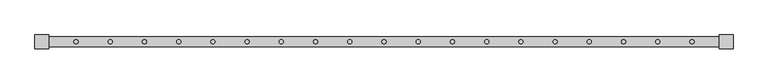
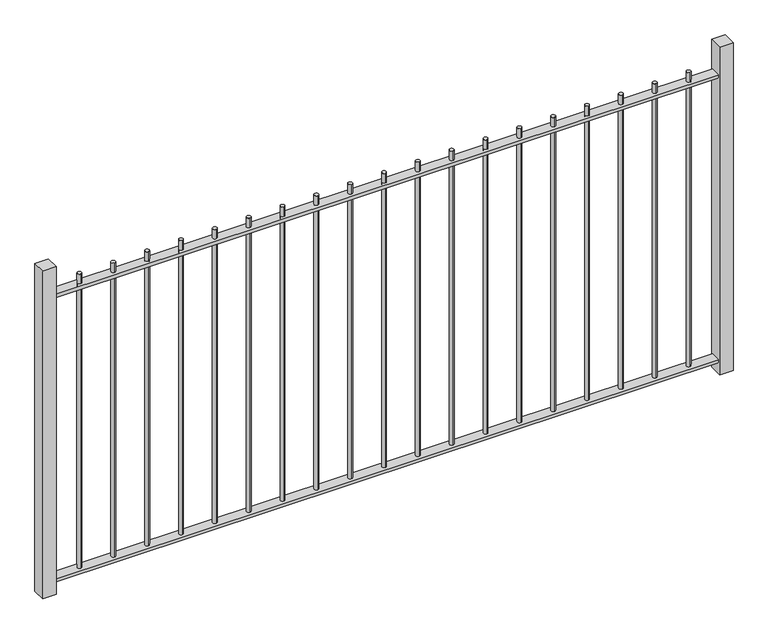
"""IFC4 building model written with IfcOpenShell, lengths in millimetres: railing geometry."""

from ifc_helpers import new_model, si_unit, point, frame, frame_2d, origin, place, context, project, spatial, polyline, circle_curve, trimmed, segment, composite_curve, outline, extrude, source, transform, mapped, element, save


def railing_b2c4460c(model_context):
    return source(origin(), model_context, "Body", "SweptSolid", [
        extrude(outline(polyline([(8650.4300877, -24901.1119119), (8650.4300877, -24961.1119119), (4650.4300877, -24961.1119119), (4650.4300877, -24901.1119119), (8650.4300877, -24901.1119119)])), frame((0.0, 0.0, -30.0), z_axis=(0.0, 0.0, 1.0), x_axis=(1.0, 0.0, 0.0)), (0.0, 0.0, 1.0), 20.0),
        extrude(outline(polyline([(8650.4300877, -24901.1119119), (8650.4300877, -24961.1119119), (4650.4300877, -24961.1119119), (4650.4300877, -24901.1119119), (8650.4300877, -24901.1119119)])), frame((0.0, 0.0, 1750.0), z_axis=(0.0, 0.0, 1.0), x_axis=(1.0, 0.0, 0.0)), (0.0, 0.0, 1.0), 20.0),
        extrude(outline(composite_curve([segment(trimmed(circle_curve(frame_2d((4850.4300877, -24931.1119119)), 12.5), [point((4850.4300877, -24943.6119119))], [point((4850.4300877, -24918.6119119))], False, "CARTESIAN"), True, "CONTINUOUS"), segment(trimmed(circle_curve(frame_2d((4850.4300877, -24931.1119119)), 12.5), [point((4850.4300877, -24918.6119119))], [point((4850.4300877, -24943.6119119))], False, "CARTESIAN"), True, "CONTINUOUS")], self_intersect=False)), frame((0.0, 0.0, -10.0), z_axis=(0.0, 0.0, 1.0), x_axis=(1.0, 0.0, 0.0)), (0.0, 0.0, 1.0), 1840.0),
        extrude(outline(composite_curve([segment(trimmed(circle_curve(frame_2d((5050.4300877, -24931.1119119)), 12.5), [point((5050.4300877, -24943.6119119))], [point((5050.4300877, -24918.6119119))], False, "CARTESIAN"), True, "CONTINUOUS"), segment(trimmed(circle_curve(frame_2d((5050.4300877, -24931.1119119)), 12.5), [point((5050.4300877, -24918.6119119))], [point((5050.4300877, -24943.6119119))], False, "CARTESIAN"), True, "CONTINUOUS")], self_intersect=False)), frame((0.0, 0.0, -10.0), z_axis=(0.0, 0.0, 1.0), x_axis=(1.0, 0.0, 0.0)), (0.0, 0.0, 1.0), 1840.0),
        extrude(outline(composite_curve([segment(trimmed(circle_curve(frame_2d((5250.4300877, -24931.1119119)), 12.5), [point((5250.4300877, -24943.6119119))], [point((5250.4300877, -24918.6119119))], False, "CARTESIAN"), True, "CONTINUOUS"), segment(trimmed(circle_curve(frame_2d((5250.4300877, -24931.1119119)), 12.5), [point((5250.4300877, -24918.6119119))], [point((5250.4300877, -24943.6119119))], False, "CARTESIAN"), True, "CONTINUOUS")], self_intersect=False)), frame((0.0, 0.0, -10.0), z_axis=(0.0, 0.0, 1.0), x_axis=(1.0, 0.0, 0.0)), (0.0, 0.0, 1.0), 1840.0),
        extrude(outline(composite_curve([segment(trimmed(circle_curve(frame_2d((5450.4300877, -24931.1119119)), 12.5), [point((5450.4300877, -24943.6119119))], [point((5450.4300877, -24918.6119119))], False, "CARTESIAN"), True, "CONTINUOUS"), segment(trimmed(circle_curve(frame_2d((5450.4300877, -24931.1119119)), 12.5), [point((5450.4300877, -24918.6119119))], [point((5450.4300877, -24943.6119119))], False, "CARTESIAN"), True, "CONTINUOUS")], self_intersect=False)), frame((0.0, 0.0, -10.0), z_axis=(0.0, 0.0, 1.0), x_axis=(1.0, 0.0, 0.0)), (0.0, 0.0, 1.0), 1840.0),
        extrude(outline(composite_curve([segment(trimmed(circle_curve(frame_2d((5650.4300877, -24931.1119119)), 12.5), [point((5650.4300877, -24943.6119119))], [point((5650.4300877, -24918.6119119))], False, "CARTESIAN"), True, "CONTINUOUS"), segment(trimmed(circle_curve(frame_2d((5650.4300877, -24931.1119119)), 12.5), [point((5650.4300877, -24918.6119119))], [point((5650.4300877, -24943.6119119))], False, "CARTESIAN"), True, "CONTINUOUS")], self_intersect=False)), frame((0.0, 0.0, -10.0), z_axis=(0.0, 0.0, 1.0), x_axis=(1.0, 0.0, 0.0)), (0.0, 0.0, 1.0), 1840.0),
        extrude(outline(composite_curve([segment(trimmed(circle_curve(frame_2d((5850.4300877, -24931.1119119)), 12.5), [point((5850.4300877, -24943.6119119))], [point((5850.4300877, -24918.6119119))], False, "CARTESIAN"), True, "CONTINUOUS"), segment(trimmed(circle_curve(frame_2d((5850.4300877, -24931.1119119)), 12.5), [point((5850.4300877, -24918.6119119))], [point((5850.4300877, -24943.6119119))], False, "CARTESIAN"), True, "CONTINUOUS")], self_intersect=False)), frame((0.0, 0.0, -10.0), z_axis=(0.0, 0.0, 1.0), x_axis=(1.0, 0.0, 0.0)), (0.0, 0.0, 1.0), 1840.0),
        extrude(outline(composite_curve([segment(trimmed(circle_curve(frame_2d((6050.4300877, -24931.1119119)), 12.5), [point((6050.4300877, -24943.6119119))], [point((6050.4300877, -24918.6119119))], False, "CARTESIAN"), True, "CONTINUOUS"), segment(trimmed(circle_curve(frame_2d((6050.4300877, -24931.1119119)), 12.5), [point((6050.4300877, -24918.6119119))], [point((6050.4300877, -24943.6119119))], False, "CARTESIAN"), True, "CONTINUOUS")], self_intersect=False)), frame((0.0, 0.0, -10.0), z_axis=(0.0, 0.0, 1.0), x_axis=(1.0, 0.0, 0.0)), (0.0, 0.0, 1.0), 1840.0),
        extrude(outline(composite_curve([segment(trimmed(circle_curve(frame_2d((6250.4300877, -24931.1119119)), 12.5), [point((6250.4300877, -24943.6119119))], [point((6250.4300877, -24918.6119119))], False, "CARTESIAN"), True, "CONTINUOUS"), segment(trimmed(circle_curve(frame_2d((6250.4300877, -24931.1119119)), 12.5), [point((6250.4300877, -24918.6119119))], [point((6250.4300877, -24943.6119119))], False, "CARTESIAN"), True, "CONTINUOUS")], self_intersect=False)), frame((0.0, 0.0, -10.0), z_axis=(0.0, 0.0, 1.0), x_axis=(1.0, 0.0, 0.0)), (0.0, 0.0, 1.0), 1840.0),
        extrude(outline(composite_curve([segment(trimmed(circle_curve(frame_2d((6450.4300877, -24931.1119119)), 12.5), [point((6450.4300877, -24943.6119119))], [point((6450.4300877, -24918.6119119))], False, "CARTESIAN"), True, "CONTINUOUS"), segment(trimmed(circle_curve(frame_2d((6450.4300877, -24931.1119119)), 12.5), [point((6450.4300877, -24918.6119119))], [point((6450.4300877, -24943.6119119))], False, "CARTESIAN"), True, "CONTINUOUS")], self_intersect=False)), frame((0.0, 0.0, -10.0), z_axis=(0.0, 0.0, 1.0), x_axis=(1.0, 0.0, 0.0)), (0.0, 0.0, 1.0), 1840.0),
        extrude(outline(composite_curve([segment(trimmed(circle_curve(frame_2d((6650.4300877, -24931.1119119)), 12.5), [point((6650.4300877, -24943.6119119))], [point((6650.4300877, -24918.6119119))], False, "CARTESIAN"), True, "CONTINUOUS"), segment(trimmed(circle_curve(frame_2d((6650.4300877, -24931.1119119)), 12.5), [point((6650.4300877, -24918.6119119))], [point((6650.4300877, -24943.6119119))], False, "CARTESIAN"), True, "CONTINUOUS")], self_intersect=False)), frame((0.0, 0.0, -10.0), z_axis=(0.0, 0.0, 1.0), x_axis=(1.0, 0.0, 0.0)), (0.0, 0.0, 1.0), 1840.0),
        extrude(outline(composite_curve([segment(trimmed(circle_curve(frame_2d((6850.4300877, -24931.1119119)), 12.5), [point((6850.4300877, -24943.6119119))], [point((6850.4300877, -24918.6119119))], False, "CARTESIAN"), True, "CONTINUOUS"), segment(trimmed(circle_curve(frame_2d((6850.4300877, -24931.1119119)), 12.5), [point((6850.4300877, -24918.6119119))], [point((6850.4300877, -24943.6119119))], False, "CARTESIAN"), True, "CONTINUOUS")], self_intersect=False)), frame((0.0, 0.0, -10.0), z_axis=(0.0, 0.0, 1.0), x_axis=(1.0, 0.0, 0.0)), (0.0, 0.0, 1.0), 1840.0),
        extrude(outline(composite_curve([segment(trimmed(circle_curve(frame_2d((7050.4300877, -24931.1119119)), 12.5), [point((7050.4300877, -24943.6119119))], [point((7050.4300877, -24918.6119119))], False, "CARTESIAN"), True, "CONTINUOUS"), segment(trimmed(circle_curve(frame_2d((7050.4300877, -24931.1119119)), 12.5), [point((7050.4300877, -24918.6119119))], [point((7050.4300877, -24943.6119119))], False, "CARTESIAN"), True, "CONTINUOUS")], self_intersect=False)), frame((0.0, 0.0, -10.0), z_axis=(0.0, 0.0, 1.0), x_axis=(1.0, 0.0, 0.0)), (0.0, 0.0, 1.0), 1840.0),
        extrude(outline(composite_curve([segment(trimmed(circle_curve(frame_2d((7250.4300877, -24931.1119119)), 12.5), [point((7250.4300877, -24943.6119119))], [point((7250.4300877, -24918.6119119))], False, "CARTESIAN"), True, "CONTINUOUS"), segment(trimmed(circle_curve(frame_2d((7250.4300877, -24931.1119119)), 12.5), [point((7250.4300877, -24918.6119119))], [point((7250.4300877, -24943.6119119))], False, "CARTESIAN"), True, "CONTINUOUS")], self_intersect=False)), frame((0.0, 0.0, -10.0), z_axis=(0.0, 0.0, 1.0), x_axis=(1.0, 0.0, 0.0)), (0.0, 0.0, 1.0), 1840.0),
        extrude(outline(composite_curve([segment(trimmed(circle_curve(frame_2d((7450.4300877, -24931.1119119)), 12.5), [point((7450.4300877, -24943.6119119))], [point((7450.4300877, -24918.6119119))], False, "CARTESIAN"), True, "CONTINUOUS"), segment(trimmed(circle_curve(frame_2d((7450.4300877, -24931.1119119)), 12.5), [point((7450.4300877, -24918.6119119))], [point((7450.4300877, -24943.6119119))], False, "CARTESIAN"), True, "CONTINUOUS")], self_intersect=False)), frame((0.0, 0.0, -10.0), z_axis=(0.0, 0.0, 1.0), x_axis=(1.0, 0.0, 0.0)), (0.0, 0.0, 1.0), 1840.0),
        extrude(outline(composite_curve([segment(trimmed(circle_curve(frame_2d((7650.4300877, -24931.1119119)), 12.5), [point((7650.4300877, -24943.6119119))], [point((7650.4300877, -24918.6119119))], False, "CARTESIAN"), True, "CONTINUOUS"), segment(trimmed(circle_curve(frame_2d((7650.4300877, -24931.1119119)), 12.5), [point((7650.4300877, -24918.6119119))], [point((7650.4300877, -24943.6119119))], False, "CARTESIAN"), True, "CONTINUOUS")], self_intersect=False)), frame((0.0, 0.0, -10.0), z_axis=(0.0, 0.0, 1.0), x_axis=(1.0, 0.0, 0.0)), (0.0, 0.0, 1.0), 1840.0),
        extrude(outline(composite_curve([segment(trimmed(circle_curve(frame_2d((7850.4300877, -24931.1119119)), 12.5), [point((7850.4300877, -24943.6119119))], [point((7850.4300877, -24918.6119119))], False, "CARTESIAN"), True, "CONTINUOUS"), segment(trimmed(circle_curve(frame_2d((7850.4300877, -24931.1119119)), 12.5), [point((7850.4300877, -24918.6119119))], [point((7850.4300877, -24943.6119119))], False, "CARTESIAN"), True, "CONTINUOUS")], self_intersect=False)), frame((0.0, 0.0, -10.0), z_axis=(0.0, 0.0, 1.0), x_axis=(1.0, 0.0, 0.0)), (0.0, 0.0, 1.0), 1840.0),
        extrude(outline(composite_curve([segment(trimmed(circle_curve(frame_2d((8050.4300877, -24931.1119119)), 12.5), [point((8050.4300877, -24943.6119119))], [point((8050.4300877, -24918.6119119))], False, "CARTESIAN"), True, "CONTINUOUS"), segment(trimmed(circle_curve(frame_2d((8050.4300877, -24931.1119119)), 12.5), [point((8050.4300877, -24918.6119119))], [point((8050.4300877, -24943.6119119))], False, "CARTESIAN"), True, "CONTINUOUS")], self_intersect=False)), frame((0.0, 0.0, -10.0), z_axis=(0.0, 0.0, 1.0), x_axis=(1.0, 0.0, 0.0)), (0.0, 0.0, 1.0), 1840.0),
        extrude(outline(composite_curve([segment(trimmed(circle_curve(frame_2d((8250.4300877, -24931.1119119)), 12.5), [point((8250.4300877, -24943.6119119))], [point((8250.4300877, -24918.6119119))], False, "CARTESIAN"), True, "CONTINUOUS"), segment(trimmed(circle_curve(frame_2d((8250.4300877, -24931.1119119)), 12.5), [point((8250.4300877, -24918.6119119))], [point((8250.4300877, -24943.6119119))], False, "CARTESIAN"), True, "CONTINUOUS")], self_intersect=False)), frame((0.0, 0.0, -10.0), z_axis=(0.0, 0.0, 1.0), x_axis=(1.0, 0.0, 0.0)), (0.0, 0.0, 1.0), 1840.0),
        extrude(outline(composite_curve([segment(trimmed(circle_curve(frame_2d((8450.4300877, -24931.1119119)), 12.5), [point((8450.4300877, -24943.6119119))], [point((8450.4300877, -24918.6119119))], False, "CARTESIAN"), True, "CONTINUOUS"), segment(trimmed(circle_curve(frame_2d((8450.4300877, -24931.1119119)), 12.5), [point((8450.4300877, -24918.6119119))], [point((8450.4300877, -24943.6119119))], False, "CARTESIAN"), True, "CONTINUOUS")], self_intersect=False)), frame((0.0, 0.0, -10.0), z_axis=(0.0, 0.0, 1.0), x_axis=(1.0, 0.0, 0.0)), (0.0, 0.0, 1.0), 1840.0),
        extrude(outline(polyline([(4690.4300877, -24891.1119119), (4690.4300877, -24971.1119119), (4610.4300877, -24971.1119119), (4610.4300877, -24891.1119119), (4690.4300877, -24891.1119119)])), frame((0.0, 0.0, -100.0), z_axis=(0.0, 0.0, 1.0), x_axis=(1.0, 0.0, 0.0)), (0.0, 0.0, 1.0), 2050.0),
        extrude(outline(polyline([(8690.4300877, -24891.1119119), (8690.4300877, -24971.1119119), (8610.4300877, -24971.1119119), (8610.4300877, -24891.1119119), (8690.4300877, -24891.1119119)])), frame((0.0, 0.0, -100.0), z_axis=(0.0, 0.0, 1.0), x_axis=(1.0, 0.0, 0.0)), (0.0, 0.0, 1.0), 2050.0),
    ])


if __name__ == "__main__":
    model = new_model("IFC4")
    model_context = context("Model", 3, world=origin())
    ifc_project = project(units=[si_unit("LENGTHUNIT", "METRE", prefix="MILLI")], contexts=[model_context])
    site = spatial("IfcSite", under=ifc_project)
    building = spatial("IfcBuilding", under=site)
    placement = place(None, origin())
    railing_shape = railing_b2c4460c(model_context)
    element("IfcRailing", 1, at=placement, inside=building, context=model_context, shape_type="MappedRepresentation", body=[
        mapped(railing_shape, transform((0.0, 0.0, 0.0), x_axis=(1.0, 0.0, 0.0), y_axis=(0.0, 1.0, 0.0), z_axis=(0.0, 0.0, 1.0))),
    ])
    save(model, "model.ifc")

# Revit data of these elements
# Element 1 (IfcRailing)
#   Materials on its faces: "NLRS_h2_staal_generiek zwart_gen_rsf", "NLRS_h2_staal_gen_rsf"
# Materials
#   "NLRS_h2_staal_generiek zwart_gen_rsf": class "Metal", colour RGB 189 187 185, transparency 0, Manufacturer = "RevitGG", URL = "www.revitgg.nl", Description = "Staal, generiek materiaal", Cost = 0
#   "NLRS_h2_staal_gen_rsf": class "H - Metaal", colour RGB 189 187 185, transparency 0, Keynote = "h2", Model = "generiek", Manufacturer = "Revit Standards Foundation", URL = "www.revitstandards.org", Description = "staal", Cost = 0
